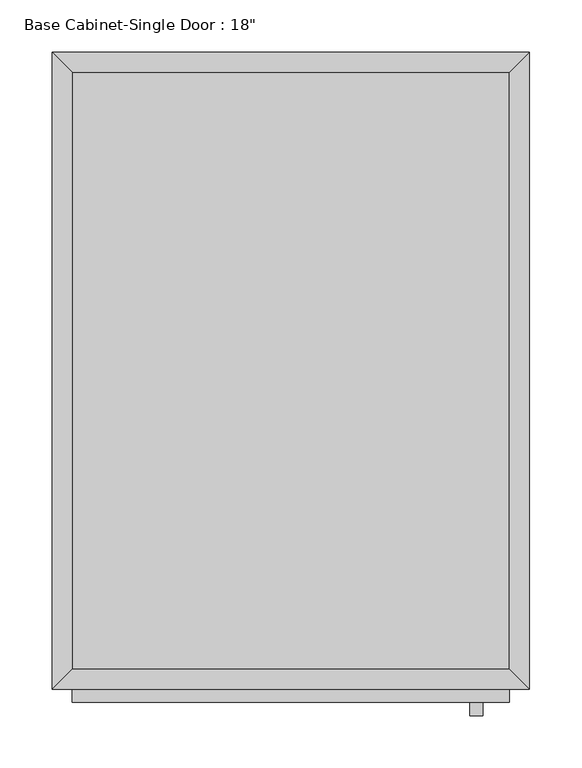
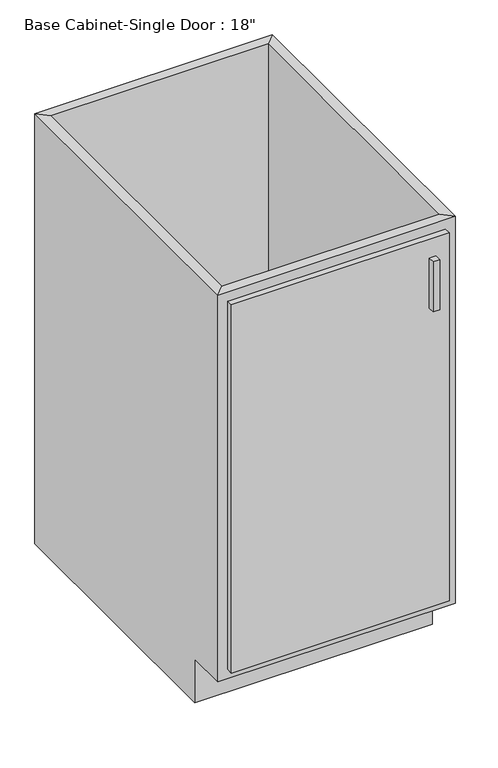
"""IFC4 building model written with IfcOpenShell, lengths in millimetres: furniture geometry."""

from ifc_helpers import new_model, si_unit, frame, origin, place, context, project, spatial, polyline, outline, extrude, faceted_brep, source, transform, mapped, element, save


def furniture_903913c9(model_context):
    return source(origin(), model_context, "Body", "SolidModel", [
        faceted_brep([(228.2877049, -590.55, 876.3), (228.2877049, -590.55, 88.9), (-190.8122951, -590.55, 88.9), (-190.8122951, -590.55, 876.3), (-209.8622951, -609.6, 876.3), (247.3377049, -609.6, 876.3), (-209.8622951, -609.6, 88.9), (247.3377049, -609.6, 88.9), (-190.8122951, -533.4, 88.9), (-190.8122951, -19.05, 88.9), (-190.8122951, -19.05, 876.3), (-209.8622951, 0.0, 876.3), (-209.8622951, 0.0, 0.0), (-209.8622951, -533.4, 0.0), (-209.8622951, -533.4, 88.9), (228.2877049, -19.05, 88.9), (228.2877049, -19.05, 876.3), (247.3377049, 0.0, 876.3), (247.3377049, 0.0, 0.0), (228.2877049, -533.4, 88.9), (247.3377049, -533.4, 88.9), (247.3377049, -533.4, 0.0)], [[[0, 1, 2, 3]], [[0, 3, 4, 5]], [[5, 4, 6, 7]], [[2, 1, 7, 6]], [[3, 2, 8, 9, 10]], [[4, 3, 10, 11]], [[6, 4, 11, 12, 13, 14]], [[2, 6, 14, 8]], [[10, 9, 15, 16]], [[11, 10, 16, 17]], [[12, 11, 17, 18]], [[1, 0, 16, 15, 19]], [[0, 5, 17, 16]], [[5, 7, 20, 21, 18, 17]], [[7, 1, 19, 20]], [[8, 19, 15, 9]], [[18, 21, 13, 12]], [[13, 21, 20, 19, 8, 14]]]),
        extrude(outline(polyline([(228.2877049, -19.05), (228.2877049, -590.55), (-190.8122951, -590.55), (-190.8122951, -19.05), (228.2877049, -19.05)])), frame((0.0, 0.0, 88.9), z_axis=(0.0, 0.0, 1.0), x_axis=(1.0, 0.0, 0.0)), (0.0, 0.0, 1.0), 19.05),
        extrude(outline(polyline([(202.8877049, -635.0), (190.1877049, -635.0), (190.1877049, -622.3), (202.8877049, -622.3), (202.8877049, -635.0)])), frame((0.0, 0.0, 717.55), z_axis=(0.0, 0.0, 1.0), x_axis=(1.0, 0.0, 0.0)), (0.0, 0.0, 1.0), 101.6),
        extrude(outline(polyline([(228.2877049, -622.3), (-190.8122951, -622.3), (-190.8122951, -609.6), (228.2877049, -609.6), (228.2877049, -622.3)])), frame((0.0, 0.0, 107.95), z_axis=(0.0, 0.0, 1.0), x_axis=(1.0, 0.0, 0.0)), (0.0, 0.0, 1.0), 749.3),
    ])


if __name__ == "__main__":
    model = new_model("IFC4")
    model_context = context("Model", 3, world=origin())
    ifc_project = project(units=[si_unit("LENGTHUNIT", "METRE", prefix="MILLI")], contexts=[model_context])
    site = spatial("IfcSite", under=ifc_project)
    building = spatial("IfcBuilding", under=site)
    placement = place(None, origin())
    furniture_shape = furniture_903913c9(model_context)
    element("IfcFurniture", 1, ObjectType="Base Cabinet-Single Door : 18\"", at=placement, inside=building, context=model_context, shape_type="MappedRepresentation", body=[
        mapped(furniture_shape, transform((0.0, 0.0, 0.0), x_axis=(1.0, 0.0, 0.0), y_axis=(0.0, 1.0, 0.0), z_axis=(0.0, 0.0, 1.0))),
    ])
    save(model, "model.ifc")

# Revit data of these elements
# Type "Base Cabinet-Single Door : 18\""
#   Assembly Code = "C1030410"
#   Depth = 2' - 0"
#   Height = 2' - 10 1/2"
#   Toe Depth = 0' - 3"
#   Toe Height = 0' - 3 1/2"
#   Width = 1' - 6"
#   Cabinet Material = Countertop & Shelf
#   Drawer Material = Countertop & Shelf
#   Handle Material = Cabinets - Handles
# Element 1 (IfcFurniture, "Base Cabinet-Single Door : 18\"")
#   Materials on its faces: "Countertop & Shelf", "Cabinets", "Cabinets - Handles"
# Materials
#   "Countertop & Shelf": class "Paint", colour RGB 76 54 29, transparency 0, Cost = 0
#   "Cabinets - Handles": class "Metal", colour RGB 57 57 57, transparency 0
#   "Cabinets": class "Miscellaneous", colour RGB 249 249 249, transparency 0
